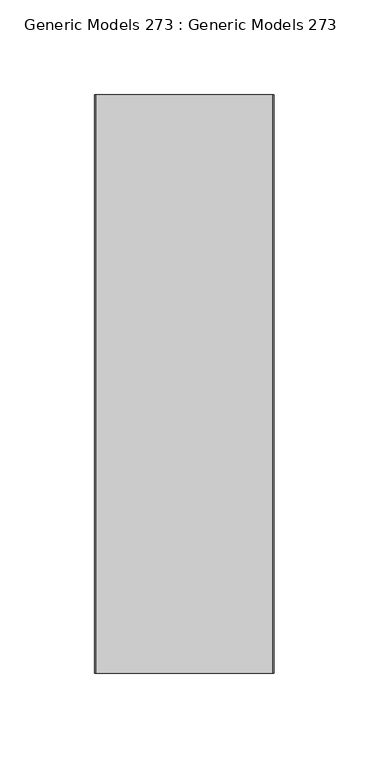
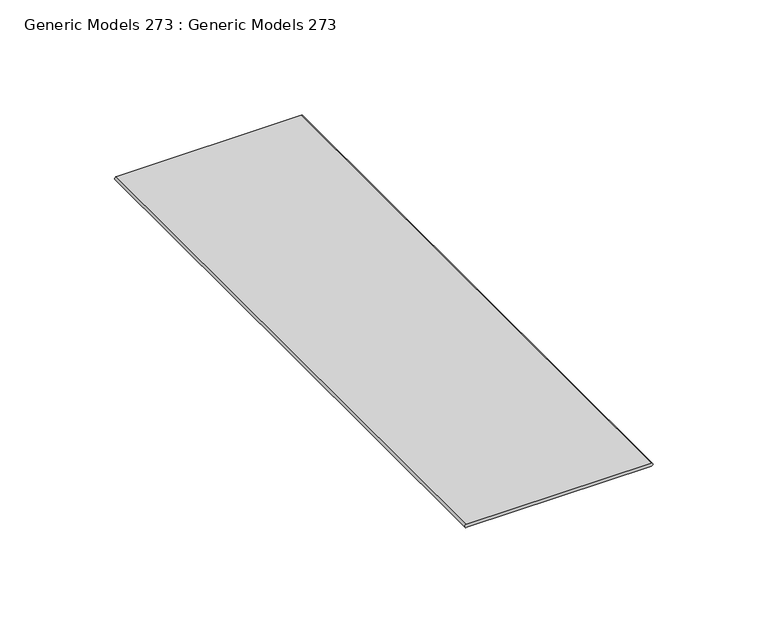
"""IFC4 building model written with IfcOpenShell, lengths in millimetres: proxy geometry, Generic Models 273 : Generic Models 273."""

from ifc_helpers import new_model, si_unit, point, frame, frame_2d, origin, place, context, project, spatial, polyline, circle_curve, trimmed, segment, composite_curve, outline, extrude, source, transform, mapped, element, save


def generic_models_273_generic_models_273_a941e2ba(model_context):
    return source(origin(), model_context, "Body", "SweptSolid", [
        extrude(outline(composite_curve([segment(trimmed(circle_curve(frame_2d((123433.1702287, 1618.0179251)), 0.79375), [point((123432.3764787, 1618.0179251))], [point((123433.9639787, 1618.0179251))], False, "CARTESIAN"), True, "CONTINUOUS"), segment(polyline([(123433.9639787, 1618.0179251), (123433.9639787, 1525.0132175)]), True, "CONTINUOUS"), segment(trimmed(circle_curve(frame_2d((123433.1702287, 1525.0132175)), 0.79375), [point((123433.9639787, 1525.0132175))], [point((123432.3764787, 1525.0132175))], False, "CARTESIAN"), True, "CONTINUOUS"), segment(polyline([(123432.3764787, 1525.0132175), (123432.3764787, 1618.0179251)]), True, "CONTINUOUS")], self_intersect=False)), frame((0.0, 4260.0872686, 0.0), z_axis=(0.0, 1.0, 0.0), x_axis=(0.0, 0.0, 1.0)), (0.0, 0.0, 1.0), 304.8),
    ])


if __name__ == "__main__":
    model = new_model("IFC4")
    model_context = context("Model", 3, world=origin())
    ifc_project = project(units=[si_unit("LENGTHUNIT", "METRE", prefix="MILLI")], contexts=[model_context])
    site = spatial("IfcSite", under=ifc_project)
    building = spatial("IfcBuilding", under=site)
    placement = place(None, origin())
    generic_models_273_generic_models_273_shape = generic_models_273_generic_models_273_a941e2ba(model_context)
    element("IfcBuildingElementProxy", 1, Name="Generic Models 273 : Generic Models 273", ObjectType="Generic Models 273 : Generic Models 273", at=placement, inside=building, context=model_context, shape_type="MappedRepresentation", body=[
        mapped(generic_models_273_generic_models_273_shape, transform((0.0, 0.0, 0.0), x_axis=(1.0, 0.0, 0.0), y_axis=(0.0, 1.0, 0.0), z_axis=(0.0, 0.0, 1.0))),
    ])
    save(model, "model.ifc")

# Revit data of these elements
# Element 1 (IfcBuildingElementProxy, "Generic Models 273 : Generic Models 273")
#   Materials on its faces: "_BED OF SEALANT"
# Materials
#   "_BED OF SEALANT": class "Generic", colour RGB 253 192 103, transparency 0, Cost = 0
